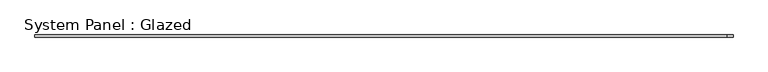
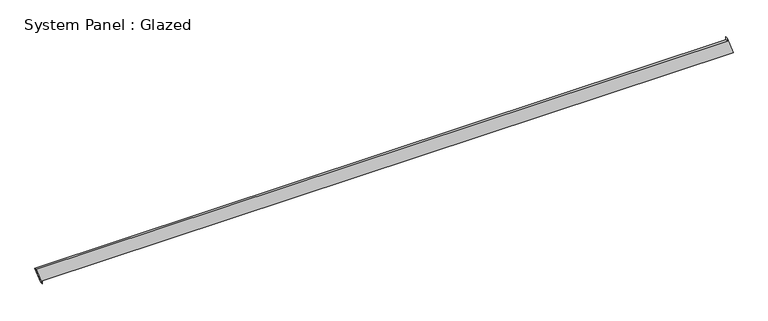
"""IFC4 building model written with IfcOpenShell, lengths in millimetres: plate geometry, System Panel : Glazed."""

from ifc_helpers import new_model, si_unit, frame, origin, place, context, project, spatial, polyline, outline, extrude, source, transform, mapped, element, save


def system_panel_glazed_eea67745(model_context):
    return source(origin(), model_context, "Body", "SweptSolid", [
        extrude(outline(polyline([(0.0, -3959.0073753), (35.3553391, -3959.0073753), (35.3553391, 4028.2307542), (235.4845779, 3958.8964427), (200.1292389, 3958.8962388), (200.1753147, -4028.2307542), (0.0, -3959.0073753)])), frame((0.0, -49.5, 0.0), z_axis=(0.0, 1.0, 0.0), x_axis=(0.0, 0.0, 1.0)), (0.0, 0.0, 1.0), 25.0),
    ])


if __name__ == "__main__":
    model = new_model("IFC4")
    model_context = context("Model", 3, world=origin())
    ifc_project = project(units=[si_unit("LENGTHUNIT", "METRE", prefix="MILLI")], contexts=[model_context])
    site = spatial("IfcSite", under=ifc_project)
    building = spatial("IfcBuilding", under=site)
    placement = place(None, origin())
    system_panel_glazed_shape = system_panel_glazed_eea67745(model_context)
    element("IfcPlate", 1, ObjectType="System Panel : Glazed", at=placement, inside=building, context=model_context, shape_type="MappedRepresentation", body=[
        mapped(system_panel_glazed_shape, transform((0.0, 0.0, 0.0), x_axis=(1.0, 0.0, 0.0), y_axis=(0.0, 1.0, 0.0), z_axis=(0.0, 0.0, 1.0))),
    ])
    save(model, "model.ifc")

# Revit data of these elements
# Element 1 (IfcPlate, "System Panel : Glazed")
#   Materials on its faces: "Glass"
# Materials
#   "Glass": class "Glass", colour RGB 218 227 224, transparency 0.85, Description = "Soda Lime Glass", Cost = 0
